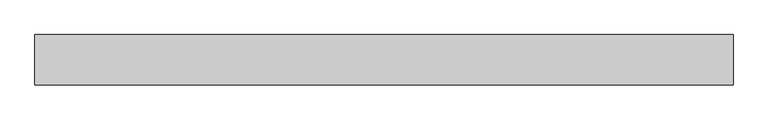
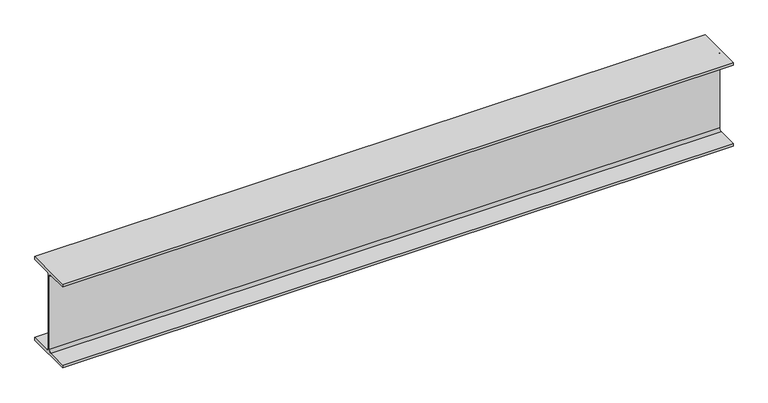
"""IFC4 building model written with IfcOpenShell, lengths in millimetres: beam geometry, Old_Steel Beam_H-KSD3502 : H_SB_ASB_H-350×175x7x11."""

from ifc_helpers import new_model, si_unit, point, frame, frame_2d, origin, place, context, project, spatial, polyline, circle_curve, trimmed, segment, composite_curve, outline, extrude, source, transform, mapped, element, save


def beam_fe8e421d(model_context):
    return source(origin(), model_context, "Body", "SweptSolid", [
        extrude(outline(composite_curve([segment(polyline([(82.5, -141.5), (82.5, -151.7), (-82.5, -151.7), (-82.5, -141.5), (-11.9, -141.5)]), True, "CONTINUOUS"), segment(trimmed(circle_curve(frame_2d((-11.9, -132.6)), 8.9), [point((-11.9, -141.5))], [point((-3.0, -132.6))], True, "CARTESIAN"), True, "CONTINUOUS"), segment(polyline([(-3.0, -132.6), (-3.0, 132.6)]), True, "CONTINUOUS"), segment(trimmed(circle_curve(frame_2d((-11.9, 132.6)), 8.9), [point((-3.0, 132.6))], [point((-11.9, 141.5))], True, "CARTESIAN"), True, "CONTINUOUS"), segment(polyline([(-11.9, 141.5), (-82.5, 141.5), (-82.5, 151.7), (82.5, 151.7), (82.5, 141.5), (11.9, 141.5)]), True, "CONTINUOUS"), segment(trimmed(circle_curve(frame_2d((11.9, 132.6)), 8.9), [point((11.9, 141.5))], [point((3.0, 132.6))], True, "CARTESIAN"), True, "CONTINUOUS"), segment(polyline([(3.0, 132.6), (3.0, -132.6)]), True, "CONTINUOUS"), segment(trimmed(circle_curve(frame_2d((11.9, -132.6)), 8.9), [point((3.0, -132.6))], [point((11.9, -141.5))], True, "CARTESIAN"), True, "CONTINUOUS"), segment(polyline([(11.9, -141.5), (82.5, -141.5)]), True, "CONTINUOUS")], self_intersect=False)), frame((-1146.3, 0.0, 0.0), z_axis=(1.0, 0.0, 0.0), x_axis=(0.0, 1.0, 0.0)), (0.0, 0.0, 1.0), 2292.6),
    ])


if __name__ == "__main__":
    model = new_model("IFC4")
    model_context = context("Model", 3, world=origin())
    ifc_project = project(units=[si_unit("LENGTHUNIT", "METRE", prefix="MILLI")], contexts=[model_context])
    site = spatial("IfcSite", under=ifc_project)
    building = spatial("IfcBuilding", under=site)
    placement = place(None, origin())
    beam_shape = beam_fe8e421d(model_context)
    element("IfcBeam", 1, ObjectType="Old_Steel Beam_H-KSD3502 : H_SB_ASB_H-350×175x7x11", at=placement, inside=building, context=model_context, shape_type="MappedRepresentation", body=[
        mapped(beam_shape, transform((0.0, 0.0, 0.0), x_axis=(1.0, 0.0, 0.0), y_axis=(0.0, 1.0, 0.0), z_axis=(0.0, 0.0, 1.0))),
    ])
    save(model, "model.ifc")

# Revit data of these elements
# Type "Old_Steel Beam_H-KSD3502 : H_SB_ASB_H-350×175x7x11"
#   Width = 17.5 cm
#   Web Thickness = 0.7 cm
#   Web Fillet = 1.4 cm
#   Warping Constant = 282290.0 cm⁶
#   Torsional Moment of Inertia = 19.4042 cm⁴
#   Torsional Modulus = 1.0 cm³
#   Section Area = 63.14 cm²
#   Plastic Modulus weak axis = 174.0 cm³
#   Plastic Modulus strong axis = 868.0 cm³
#   Perimeter = 1.36 m²/m
#   Nominal Weight = 49.60 kgf/m
#   Moment of Inertia weak axis = 984.00 cm⁴
#   Moment of Inertia strong axis = 13600.00 cm⁴
#   Height = 35.0 cm
#   Flange Thickness = 1.1 cm
#   Elastic Modulus weak axis = 112.0 cm³
#   Elastic Modulus strong axis = 775.0 cm³
#   Centroid Vertical = 17.5 cm
#   Centroid Horizontal = 8.75 cm
#   Length [instance default] = 1.5240 m
#   Structural Material [instance default] = Steel, 45-345
#   Assembly Code = ""
# Element 1 (IfcBeam, "Old_Steel Beam_H-KSD3502 : H_SB_ASB_H-350×175x7x11")
#   Structural Material = none
# Materials
#   "Steel, 45-345": class "Metal", colour RGB 189 187 185, transparency 0, Description = "Steel 345 MPa", Cost = 0
